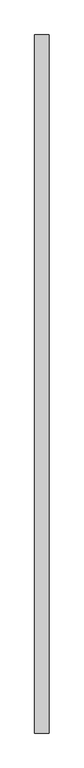
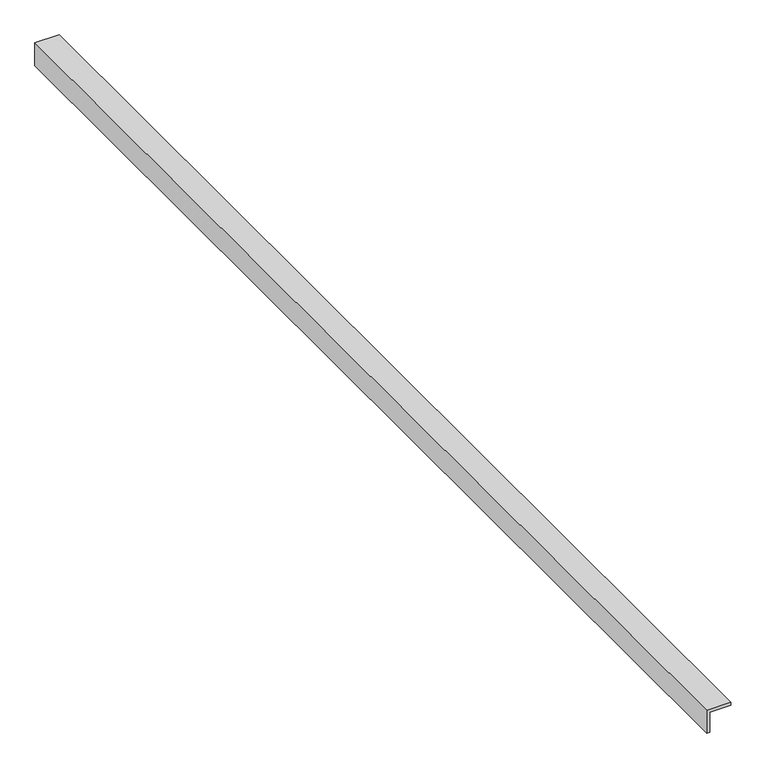
"""IFC4 building model written with IfcOpenShell, lengths in millimetres: proxy geometry, Generic Models 3:Generic Models 2:312240:Generic Models 2:312240 : Generic Models 3:Generic Models 2:312240:6 : Generic Models 3:Generic Models 2:312240:Generic Models 2:312240 : Generic Models 3:Generic Models 2:312240:300533."""

from ifc_helpers import new_model, si_unit, frame, origin, place, context, project, spatial, polyline, outline, extrude, source, transform, mapped, element, save


def generic_models_3ae80ee4(model_context):
    return source(origin(), model_context, "Body", "SweptSolid", [
        extrude(outline(polyline([(-28.575, 667585.4117239), (-79.375, 667585.4117239), (-79.375, 667591.7617239), (-34.925, 667591.7617239), (-34.925, 667636.2117239), (-28.575, 667636.2117239), (-28.575, 667585.4117239)])), frame((0.0, -568496.2038841, 0.0), z_axis=(0.0, 1.0, 0.0), x_axis=(0.0, 0.0, 1.0)), (0.0, 0.0, 1.0), 2438.4),
    ])


if __name__ == "__main__":
    model = new_model("IFC4")
    model_context = context("Model", 3, world=origin())
    ifc_project = project(units=[si_unit("LENGTHUNIT", "METRE", prefix="MILLI")], contexts=[model_context])
    site = spatial("IfcSite", under=ifc_project)
    building = spatial("IfcBuilding", under=site)
    placement = place(None, origin())
    generic_models_shape = generic_models_3ae80ee4(model_context)
    element("IfcBuildingElementProxy", 1, Name="Generic Models 3:Generic Models 2:312240:Generic Models 2:312240 : Generic Models 3:Generic Models 2:312240:6 : Generic Models 3:Generic Models 2:312240:Generic Models 2:312240 : Generic Models 3:Generic Models 2:312240:300533", ObjectType="Generic Models 3:Generic Models 2:312240:Generic Models 2:312240 : Generic Models 3:Generic Models 2:312240:6 : Generic Models 3:Generic Models 2:312240:Generic Models 2:312240 : Generic Models 3:Generic Models 2:312240:300533", at=placement, inside=building, context=model_context, shape_type="MappedRepresentation", body=[
        mapped(generic_models_shape, transform((0.0, 0.0, 0.0), x_axis=(1.0, 0.0, 0.0), y_axis=(0.0, 1.0, 0.0), z_axis=(0.0, 0.0, 1.0))),
    ])
    save(model, "model.ifc")

# Revit data of these elements
# Type "Generic Models 3:Generic Models 2:312240:Generic Models 2:312240 : Generic Models 3:Generic Models 2:312240:6 : Generic Models 3:Generic Models 2:312240:Generic Models 2:312240 : Generic Models 3:Generic Models 2:312240:300533"
#   NameOverride = "Generic Models 3:Generic Models 2:312240:Generic Models 2:312240 : Generic Models 3:Generic Models 2:312240:300533"
#   ObjectTypeOverride = "Generic Models 2:312240 : Generic Models 3:Generic Models 2:312240"
#   Reference = "Generic Models 2"
#   Tag = "300533"
# Element 1 (IfcBuildingElementProxy, "Generic Models 3:Generic Models 2:312240:Generic Models 2:312240 : Generic Models 3:Generic Models 2:312240:6 : Generic Models 3:Generic Models 2:312240:Generic Models 2:312240 : Generic Models 3:Generic Models 2:312240:300533")
#   Materials on its faces: "GALVANIZED STEEL ANGLE (L2x2x1/4) - 1/4\" HILTI KWIK HUS-EZ W/ MIN EMBED=2-1/2\" @ 24\""
# Materials
#   "GALVANIZED STEEL ANGLE (L2x2x1/4) - 1/4\" HILTI KWIK HUS-EZ W/ MIN EMBED=2-1/2\" @ 24\"": class "Unassigned", colour RGB 210 209 208, transparency 0, Keynote = "M05121300.02", Cost = 0
